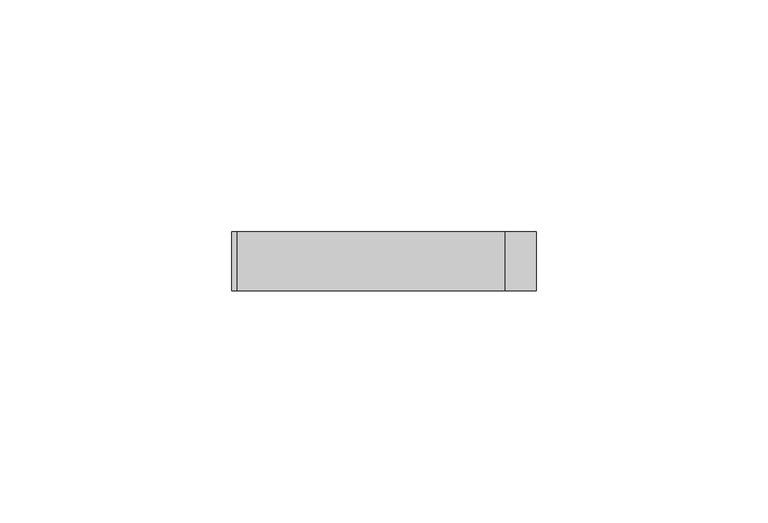
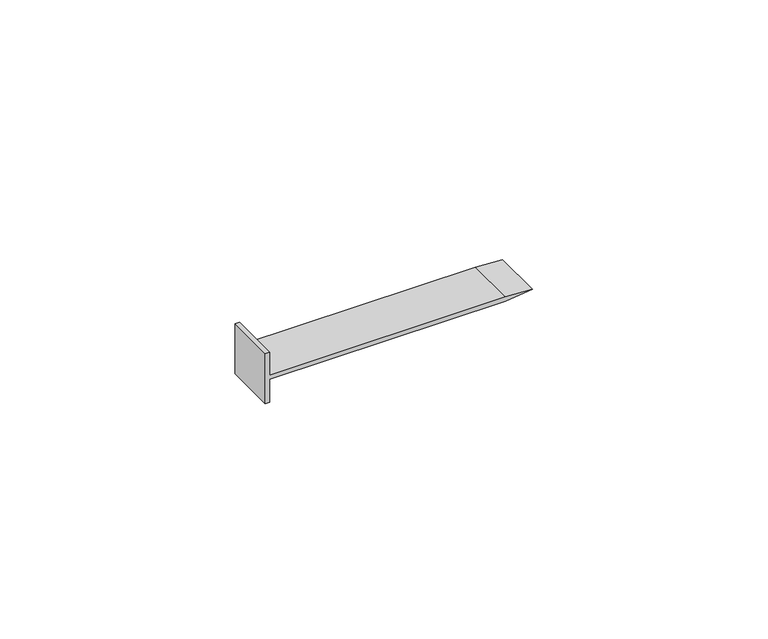
"""IFC4 building model written with IfcOpenShell, lengths in millimetres: proxy geometry, STAINLESS STEEL NAILS011 15348 : STAINLESS STEEL NAILS011 15348."""

from ifc_helpers import new_model, si_unit, frame, origin, place, context, project, spatial, polyline, outline, extrude, source, transform, mapped, element, save


def generic_models_33362b51(model_context):
    return source(origin(), model_context, "Body", "SweptSolid", [
        extrude(outline(polyline([(40201.6774651, -2780.8277654), (40201.6774651, -2779.7445667), (40207.6350577, -2779.7445667), (40207.6350577, -2721.8057893), (40208.3564507, -2715.1766231), (40208.7182563, -2721.8057893), (40208.7182563, -2779.7445667), (40214.675849, -2779.7445667), (40214.675849, -2780.8277654), (40201.6774651, -2780.8277654)])), frame((0.0, -1065.5906573, 0.0), z_axis=(0.0, 1.0, 0.0), x_axis=(0.0, 0.0, 1.0)), (0.0, 0.0, 1.0), 12.7),
    ])


if __name__ == "__main__":
    model = new_model("IFC4")
    model_context = context("Model", 3, world=origin())
    ifc_project = project(units=[si_unit("LENGTHUNIT", "METRE", prefix="MILLI")], contexts=[model_context])
    site = spatial("IfcSite", under=ifc_project)
    building = spatial("IfcBuilding", under=site)
    placement = place(None, origin())
    generic_models_shape = generic_models_33362b51(model_context)
    element("IfcBuildingElementProxy", 1, Name="STAINLESS STEEL NAILS011 15348 : STAINLESS STEEL NAILS011 15348", ObjectType="STAINLESS STEEL NAILS011 15348 : STAINLESS STEEL NAILS011 15348", at=placement, inside=building, context=model_context, shape_type="MappedRepresentation", body=[
        mapped(generic_models_shape, transform((0.0, 0.0, 0.0), x_axis=(1.0, 0.0, 0.0), y_axis=(0.0, 1.0, 0.0), z_axis=(0.0, 0.0, 1.0))),
    ])
    save(model, "model.ifc")

# Revit data of these elements
# Type "STAINLESS STEEL NAILS011 15348 : STAINLESS STEEL NAILS011 15348"
#   NameOverride = "STAINLESS STEEL NAILS011"
# Element 1 (IfcBuildingElementProxy, "STAINLESS STEEL NAILS011 15348 : STAINLESS STEEL NAILS011 15348")
#   Materials on its faces: "1 3/4\" STAINLESS STEEL RINGSHANK 5D COMMON NAILS @ 4\" (101.6MM) O.C. FIRESTONE PROVIDED MAX., 1/2\" STAGGERED"
# Materials
#   "1 3/4\" STAINLESS STEEL RINGSHANK 5D COMMON NAILS @ 4\" (101.6MM) O.C. FIRESTONE PROVIDED MAX., 1/2\" STAGGERED": class "Unassigned", colour RGB 255 255 255, transparency 0
